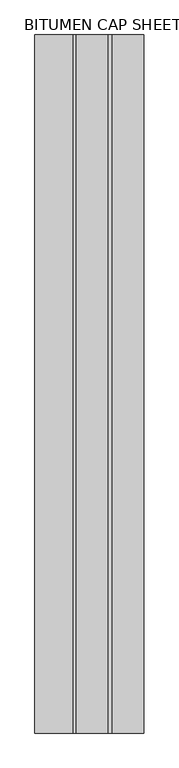
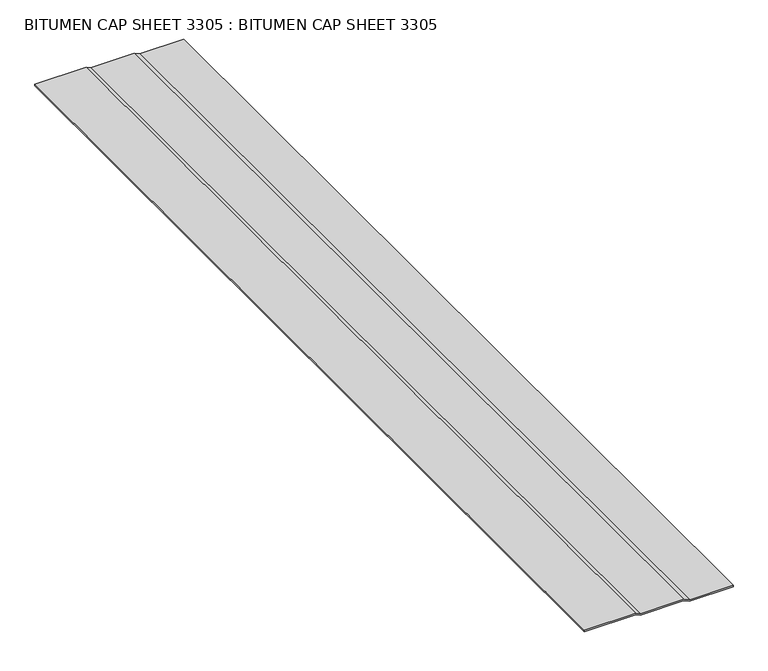
"""IFC4 building model written with IfcOpenShell, lengths in millimetres: proxy geometry, BITUMEN CAP SHEET 3305 : BITUMEN CAP SHEET 3305."""

from ifc_helpers import new_model, si_unit, frame, origin, place, context, project, spatial, polyline, outline, extrude, source, transform, mapped, element, save


def bitumen_cap_sheet_3305_bitumen_cap_sheet_3305_313e2dc3(model_context):
    return source(origin(), model_context, "Body", "SweptSolid", [
        extrude(outline(polyline([(40259.2002678, -2469.2761954), (40262.3752678, -2469.2761954), (40262.3752678, -2560.795457), (40267.6612773, -2573.2602756), (40267.6612773, -2663.9440313), (40271.9940719, -2673.6609328), (40271.9940719, -2781.5474293), (40268.8188423, -2781.5474293), (40268.8188423, -2674.3362183), (40264.4862773, -2664.6198318), (40264.4862773, -2573.9056756), (40259.2002678, -2561.440857), (40259.2002678, -2469.2761954)])), frame((0.0, -1052.8906574, 0.0), z_axis=(0.0, 1.0, 0.0), x_axis=(0.0, 0.0, 1.0)), (0.0, 0.0, 1.0), 2000.25),
    ])


if __name__ == "__main__":
    model = new_model("IFC4")
    model_context = context("Model", 3, world=origin())
    ifc_project = project(units=[si_unit("LENGTHUNIT", "METRE", prefix="MILLI")], contexts=[model_context])
    site = spatial("IfcSite", under=ifc_project)
    building = spatial("IfcBuilding", under=site)
    placement = place(None, origin())
    bitumen_cap_sheet_3305_bitumen_cap_sheet_3305_shape = bitumen_cap_sheet_3305_bitumen_cap_sheet_3305_313e2dc3(model_context)
    element("IfcBuildingElementProxy", 1, Name="BITUMEN CAP SHEET 3305 : BITUMEN CAP SHEET 3305", ObjectType="BITUMEN CAP SHEET 3305 : BITUMEN CAP SHEET 3305", at=placement, inside=building, context=model_context, shape_type="MappedRepresentation", body=[
        mapped(bitumen_cap_sheet_3305_bitumen_cap_sheet_3305_shape, transform((0.0, 0.0, 0.0), x_axis=(1.0, 0.0, 0.0), y_axis=(0.0, 1.0, 0.0), z_axis=(0.0, 0.0, 1.0))),
    ])
    save(model, "model.ifc")

# Revit data of these elements
# Type "BITUMEN CAP SHEET 3305 : BITUMEN CAP SHEET 3305"
#   NameOverride = "BITUMEN CAP SHEET"
# Element 1 (IfcBuildingElementProxy, "BITUMEN CAP SHEET 3305 : BITUMEN CAP SHEET 3305")
#   Materials on its faces: "MODIFIED BITUMEN GRANULE SURFACED CAP SHEET"
# Materials
#   "MODIFIED BITUMEN GRANULE SURFACED CAP SHEET": class "Unassigned", colour RGB 85 85 127, transparency 0
